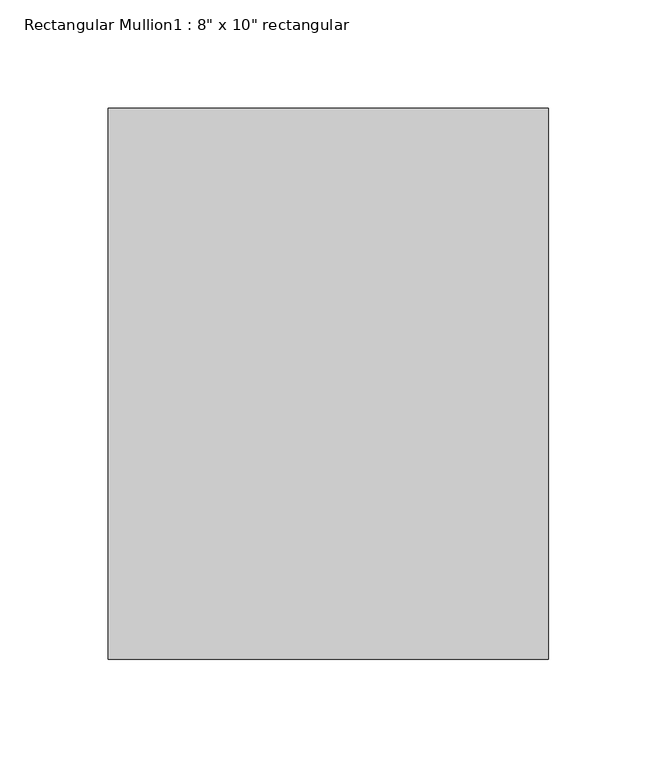
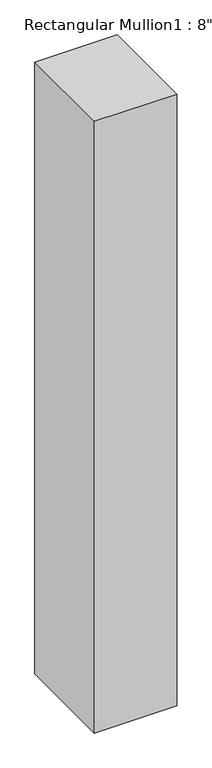
"""IFC4 building model written with IfcOpenShell, lengths in millimetres: member geometry."""

from ifc_helpers import new_model, si_unit, frame, origin, place, context, project, spatial, polyline, outline, extrude, source, transform, mapped, element, save


def member_b2bf14c7(model_context):
    return source(origin(), model_context, "Body", "SweptSolid", [
        extrude(outline(polyline([(101.6, 127.0), (101.6, -127.0), (-101.6, -127.0), (-101.6, 127.0), (101.6, 127.0)])), frame((0.0, 0.0, -1593.8500097), z_axis=(0.0, 0.0, 1.0), x_axis=(1.0, 0.0, 0.0)), (0.0, 0.0, 1.0), 1593.8500097),
    ])


if __name__ == "__main__":
    model = new_model("IFC4")
    model_context = context("Model", 3, world=origin())
    ifc_project = project(units=[si_unit("LENGTHUNIT", "METRE", prefix="MILLI")], contexts=[model_context])
    site = spatial("IfcSite", under=ifc_project)
    building = spatial("IfcBuilding", under=site)
    placement = place(None, origin())
    member_shape = member_b2bf14c7(model_context)
    element("IfcMember", 1, ObjectType="Rectangular Mullion1 : 8\" x 10\" rectangular", at=placement, inside=building, context=model_context, shape_type="MappedRepresentation", body=[
        mapped(member_shape, transform((0.0, 0.0, 0.0), x_axis=(1.0, 0.0, 0.0), y_axis=(0.0, 1.0, 0.0), z_axis=(0.0, 0.0, 1.0))),
    ])
    save(model, "model.ifc")

# Revit data of these elements
# Type "Rectangular Mullion1 : 8\" x 10\" rectangular"
#   built-in parameter 1007304 = 0.833333 (stored number, unit not read)
#   built-in parameter 1007301 = 0.333333 (stored number, unit not read)
#   built-in parameter 1007300 = 0.333333 (stored number, unit not read)
# Element 1 (IfcMember, "Rectangular Mullion1 : 8\" x 10\" rectangular")
#   Materials on its faces: "support-frame"
# Materials
#   "support-frame": class "Unassigned", colour RGB 233 233 233, transparency 0, Cost = 0
